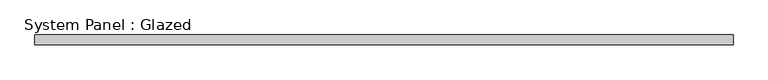
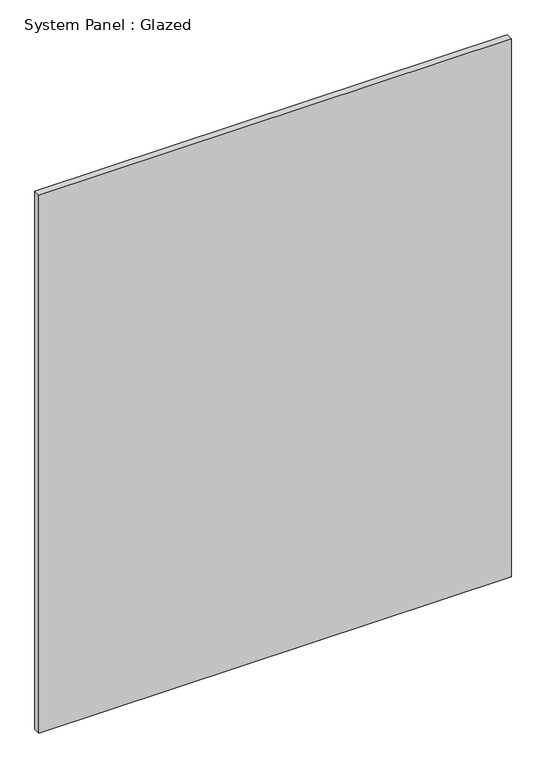
"""IFC4 building model written with IfcOpenShell, lengths in millimetres: plate geometry, System Panel : Glazed."""

import ifcopenshell
import ifcopenshell.guid

model = None  # the IFC model being written
_history = None  # IfcOwnerHistory: only IFC2X3 demands one
_inside = {}  # id of a spatial element -> (the spatial element, [elements in it])
_under = {}  # id of a project, library or spatial element -> (it, [spatial elements below it])
_declared = {}  # id of a project -> (the project, [libraries it declares])
_typed = {}  # id of a type object -> (the type object, [elements of that type])
_made_of = {}  # id of a material, layer set ... -> (it, [elements and type objects made of it])


def new_model(schema):
    """Start an empty IFC model of exactly this schema.

    Asked for "IFC4X3", IfcOpenShell would pick the latest addendum, in which some entities
    have other attributes; the version numbers below select the first issue.
    IFC2X3 requires an IfcOwnerHistory on every rooted entity: one is made here for all.
    """
    global model, _history
    if schema == "IFC4X3":
        model = ifcopenshell.file(schema_version=(4, 3, 0, 0))
    else:
        model = ifcopenshell.file(schema=schema)
    _inside.clear()
    _under.clear()
    _declared.clear()
    _typed.clear()
    _made_of.clear()
    _history = None
    if model.schema == "IFC2X3":
        org = make("IfcOrganization", Name="unknown")
        user = make(
            "IfcPersonAndOrganization",
            ThePerson=make("IfcPerson", FamilyName="unknown"),
            TheOrganization=org,
        )
        app = make(
            "IfcApplication",
            ApplicationDeveloper=org,
            Version="unknown",
            ApplicationFullName="unknown",
            ApplicationIdentifier="unknown",
        )
        _history = make(
            "IfcOwnerHistory",
            OwningUser=user,
            OwningApplication=app,
            ChangeAction="ADDED",
            CreationDate=0,
        )
    return model


def make(cls, **values):
    """One entity of the class cls with the attributes given. An attribute that is None is left unset."""
    return model.create_entity(
        cls, **{name: value for name, value in values.items() if value is not None}
    )


def rooted(cls, **values):
    """An entity with a GlobalId (a new one), such as an element, a storey or a relation."""
    return make(cls, GlobalId=ifcopenshell.guid.new(), OwnerHistory=_history, **values)


def si_unit(unit_type, name, prefix=None):
    """IfcSIUnit, for example si_unit("LENGTHUNIT", "METRE", prefix="MILLI")."""
    return make("IfcSIUnit", UnitType=unit_type, Prefix=prefix, Name=name)


def assignment(units):
    """IfcUnitAssignment: the units of a project."""
    return None if units is None else make("IfcUnitAssignment", Units=units)


def point(xyz):
    """IfcCartesianPoint."""
    return None if xyz is None else make("IfcCartesianPoint", Coordinates=xyz)


def direction(xyz):
    """IfcDirection."""
    return None if xyz is None else make("IfcDirection", DirectionRatios=xyz)


def frame(location, z_axis=None, x_axis=None):
    """IfcAxis2Placement3D, a coordinate frame: its origin and axes. An axis left out is left unset."""
    return make(
        "IfcAxis2Placement3D",
        Location=point(location),
        Axis=direction(z_axis),
        RefDirection=direction(x_axis),
    )


def origin():
    """The frame at (0, 0, 0) with its axes left unset."""
    return frame((0.0, 0.0, 0.0))


def origin_with_axes():
    """The frame at (0, 0, 0) with the z axis (0, 0, 1) and the x axis (1, 0, 0) written out."""
    return frame((0.0, 0.0, 0.0), z_axis=(0.0, 0.0, 1.0), x_axis=(1.0, 0.0, 0.0))


def place(relative_to, where):
    """IfcLocalPlacement: puts the frame where relative to a parent placement (None: the world)."""
    return make(
        "IfcLocalPlacement", PlacementRelTo=relative_to, RelativePlacement=where
    )


def context(
    kind, dimensions, precision=None, world=None, true_north=None, identifier=None
):
    """IfcGeometricRepresentationContext, for example the 3D "Model" context."""
    return make(
        "IfcGeometricRepresentationContext",
        ContextIdentifier=identifier,
        ContextType=kind,
        CoordinateSpaceDimension=dimensions,
        Precision=precision,
        WorldCoordinateSystem=world,
        TrueNorth=true_north,
    )


def project(units=None, contexts=None):
    """IfcProject with its units and contexts."""
    return rooted(
        "IfcProject",
        Name="project",
        RepresentationContexts=contexts,
        UnitsInContext=assignment(units),
    )


def spatial(cls, under=None, at=None, **own):
    """A site, building, storey or space (cls), placed at a placement, below another one or the project."""
    s = rooted(cls, ObjectPlacement=at, **own)
    if under is not None:
        _under.setdefault(under.id(), (under, []))[1].append(s)
    return s


def polyline(points):
    """IfcPolyline through the points."""
    return make("IfcPolyline", Points=[point(p) for p in points])


def outline(outer, holes=None, kind="AREA"):
    """IfcArbitraryClosedProfileDef: a profile drawn as a closed curve; with holes, ...WithVoids."""
    if holes is None:
        return make("IfcArbitraryClosedProfileDef", ProfileType=kind, OuterCurve=outer)
    return make(
        "IfcArbitraryProfileDefWithVoids",
        ProfileType=kind,
        OuterCurve=outer,
        InnerCurves=holes,
    )


def extrude(swept, where, along, depth):
    """IfcExtrudedAreaSolid: the profile swept, set in the frame where, extruded along a direction by depth."""
    return make(
        "IfcExtrudedAreaSolid",
        SweptArea=swept,
        Position=where,
        ExtrudedDirection=direction(along),
        Depth=depth,
    )


def shape(context_of_items, identifier, shape_type, items):
    """IfcShapeRepresentation: the items that make up one representation, for example the "Body"."""
    return make(
        "IfcShapeRepresentation",
        ContextOfItems=context_of_items,
        RepresentationIdentifier=identifier,
        RepresentationType=shape_type,
        Items=items,
    )


def source(mapping_origin, context_of_items, identifier, shape_type, items):
    """IfcRepresentationMap: a shape defined once, which mapped items show again and again."""
    return make(
        "IfcRepresentationMap",
        MappingOrigin=mapping_origin,
        MappedRepresentation=shape(context_of_items, identifier, shape_type, items),
    )


def transform(
    local_origin,
    x_axis=None,
    y_axis=None,
    z_axis=None,
    scale=None,
    scale2=None,
    scale3=None,
    uniform=True,
):
    """IfcCartesianTransformationOperator3D, or its non-uniform kind. x_axis, y_axis, z_axis: its Axis1, 2, 3."""
    if uniform:
        return make(
            "IfcCartesianTransformationOperator3D",
            Axis1=direction(x_axis),
            Axis2=direction(y_axis),
            LocalOrigin=point(local_origin),
            Scale=scale,
            Axis3=direction(z_axis),
        )
    return make(
        "IfcCartesianTransformationOperator3DnonUniform",
        Axis1=direction(x_axis),
        Axis2=direction(y_axis),
        LocalOrigin=point(local_origin),
        Scale=scale,
        Axis3=direction(z_axis),
        Scale2=scale2,
        Scale3=scale3,
    )


def mapped(mapping_source, mapping_target):
    """IfcMappedItem: shows the shape of a source again, moved by a transform."""
    return make(
        "IfcMappedItem", MappingSource=mapping_source, MappingTarget=mapping_target
    )


def made_of(thing, what):
    """Note that an element or type object is made of a material, layer set ...; save() writes the relation."""
    if what is not None:
        _made_of.setdefault(what.id(), (what, []))[1].append(thing)
    return thing


def element(
    cls,
    number,
    at=None,
    inside=None,
    cuts=None,
    type_object=None,
    material=None,
    context=None,
    identifier="Body",
    shape_type=None,
    held_by="IfcProductDefinitionShape",
    body=None,
    shapes=None,
    **own,
):
    """One element of the class cls, such as IfcWall. Its Tag is "e" and its number.

    at: its placement. inside: the storey or other place that contains it. cuts: it is an
    opening in that element (IfcRelVoidsElement). A single representation is given by context,
    identifier, shape_type and body (its items); several are given by shapes. held_by: the class
    of the entity that holds the representations. save() writes the other relations.
    """
    e = rooted(cls, Tag="e%d" % number, ObjectPlacement=at, **own)
    if body is not None:
        shapes = [shape(context, identifier, shape_type, body)]
    if shapes is not None:
        e.Representation = make(held_by, Representations=shapes)
    if inside is not None:
        _inside.setdefault(inside.id(), (inside, []))[1].append(e)
    if cuts is not None:
        rooted(
            "IfcRelVoidsElement", RelatingBuildingElement=cuts, RelatedOpeningElement=e
        )
    if type_object is not None:
        _typed.setdefault(type_object.id(), (type_object, []))[1].append(e)
    return made_of(e, material)


def aggregate(whole, parts):
    """IfcRelAggregates: a whole, such as a stair, and the parts it consists of."""
    return rooted("IfcRelAggregates", RelatingObject=whole, RelatedObjects=parts)


def save(model, path):
    """Write the relations noted so far, then the file.

    IfcRelAggregates (storeys below a building ...), IfcRelContainedInSpatialStructure (elements
    in a storey), IfcRelDefinesByType, IfcRelAssociatesMaterial and IfcRelDeclares: one each for
    every whole, place, type object, material and project.
    """
    for whole, parts in _under.values():
        aggregate(whole, parts)
    for where, things in _inside.values():
        rooted(
            "IfcRelContainedInSpatialStructure",
            RelatedElements=things,
            RelatingStructure=where,
        )
    for kind, things in _typed.values():
        rooted("IfcRelDefinesByType", RelatedObjects=things, RelatingType=kind)
    for what, things in _made_of.values():
        rooted("IfcRelAssociatesMaterial", RelatedObjects=things, RelatingMaterial=what)
    for by, libraries in _declared.values():
        rooted("IfcRelDeclares", RelatingContext=by, RelatedDefinitions=libraries)
    model.write(path)


def system_panel_glazed_2a5f5069(model_context):
    return source(origin(), model_context, "Body", "SweptSolid", [
        extrude(outline(polyline([(883.5, -49.5), (-883.5, -49.5), (-883.5, -24.5), (883.5, -24.5), (883.5, -49.5)])), origin_with_axes(), (0.0, 0.0, 1.0), 2125.0),
    ])


if __name__ == "__main__":
    model = new_model("IFC4")
    model_context = context("Model", 3, world=origin())
    ifc_project = project(units=[si_unit("LENGTHUNIT", "METRE", prefix="MILLI")], contexts=[model_context])
    site = spatial("IfcSite", under=ifc_project)
    building = spatial("IfcBuilding", under=site)
    placement = place(None, origin())
    system_panel_glazed_shape = system_panel_glazed_2a5f5069(model_context)
    element("IfcPlate", 1, ObjectType="System Panel : Glazed", at=placement, inside=building, context=model_context, shape_type="MappedRepresentation", body=[
        mapped(system_panel_glazed_shape, transform((0.0, 0.0, 0.0), x_axis=(1.0, 0.0, 0.0), y_axis=(0.0, 1.0, 0.0), z_axis=(0.0, 0.0, 1.0))),
    ])
    save(model, "model.ifc")

# Revit data of these elements
# Type "System Panel : Glazed"
#   Keynote = "H11"
#   Construction Type Id = "GSP4R"
#   Analytic Construction = "1/8 in Pilkington single glazing"
#   Visual Light Transmittance = 0.9
#   Solar Heat Gain Coefficient = 0.86
#   Heat Transfer Coefficient (U) = 6.7069 W/(m²·K)
# Element 1 (IfcPlate, "System Panel : Glazed")
#   Materials on its faces: "Glass"
# Materials
#   "Glass": class "Glass", colour RGB 0 128 192, transparency 0.9, Description = "Soda Lime Glass", Cost = 0
